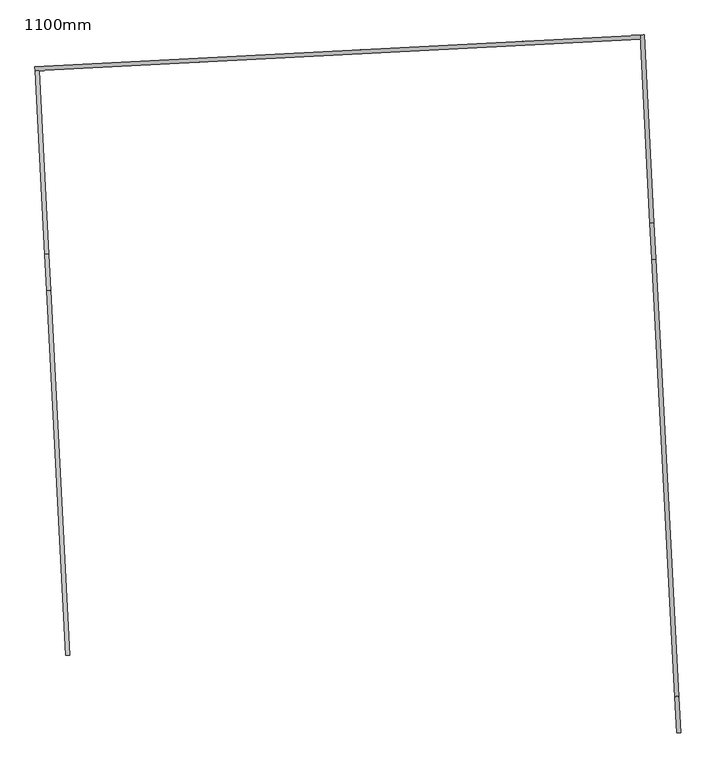
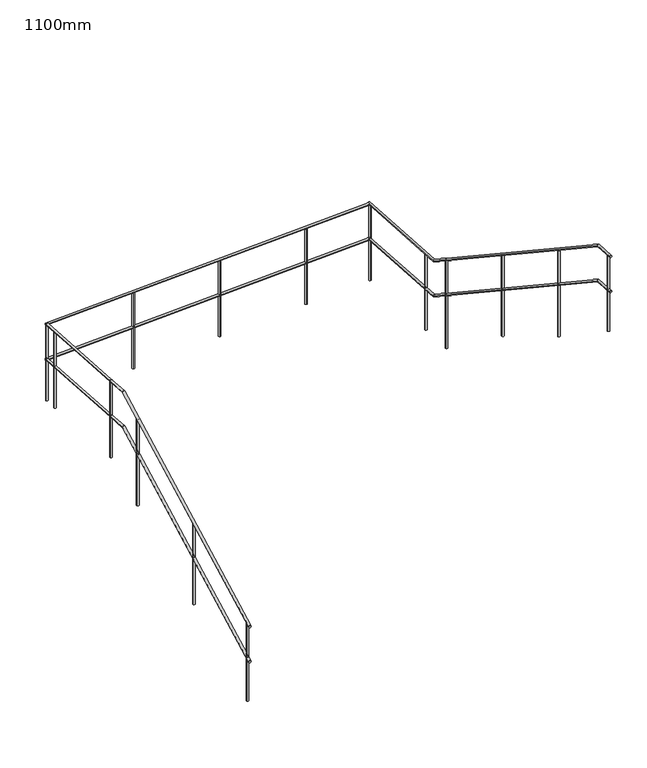
"""IFC4 building model written with IfcOpenShell, lengths in millimetres: railing geometry, 1100mm."""

from ifc_helpers import new_model, si_unit, point, frame, frame_2d, origin, place, context, project, spatial, circle_curve, ellipse_curve, trimmed, segment, composite_curve, outline, extrude, source, transform, mapped, element, save
from ifc_brep_helpers import plane_surface, cylinder_surface, advanced_brep


def railing_1100mm_925ff370(model_context):
    return source(origin(), model_context, "Body", "SolidModel", [
        advanced_brep(
        [(21553.8210897, 12464.3641407, 457.1248327), (21523.8622036, 12462.794062, 457.1248327), (21412.281847, 15165.0937775, 2210.0), (21382.3229609, 15163.5236988, 2210.0), (21398.3832997, 15430.2938589, 2210.0), (21368.4244136, 15428.7237802, 2210.0)],
        [
            (0, 1, ellipse_curve(frame((21538.8416467, 12463.5791013, 457.1248327), z_axis=(0.052335956242941364, -0.998629534754574, 0.0), x_axis=(0.0, 0.0, -1.0)), 17.8751673, 15.0)),
            (1, 0, ellipse_curve(frame((21538.8416467, 12463.5791013, 457.1248327), z_axis=(0.052335956242941364, -0.998629534754574, 0.0), x_axis=(0.0, 0.0, -1.0)), 17.8751673, 15.0)),
            (0, 2),
            (2, 3, ellipse_curve(frame((21397.302404, 15164.3087382, 2210.0), z_axis=(0.05018733030882, -0.957631309614881, -0.28359038545367027), x_axis=(-0.014841974004008681, 0.2832017346864693, -0.9589455111101147)), 15.6421818, 15.0)),
            (3, 1),
            (3, 2, ellipse_curve(frame((21397.302404, 15164.3087382, 2210.0), z_axis=(0.05018733030882, -0.957631309614881, -0.28359038545367027), x_axis=(-0.014841974004008681, 0.2832017346864693, -0.9589455111101147)), 15.6421818, 15.0)),
            (4, 5, circle_curve(frame((21383.4038566, 15429.5088195, 2210.0), z_axis=(-0.05233595624293373, 0.9986295347545745, 0.0), x_axis=(-0.9986295347545745, -0.05233595624293373, 0.0)), 15.0)),
            (5, 4, circle_curve(frame((21383.4038566, 15429.5088195, 2210.0), z_axis=(-0.05233595624293373, 0.9986295347545745, 0.0), x_axis=(-0.9986295347545745, -0.05233595624293373, 0.0)), 15.0)),
            (2, 4),
            (5, 3),
        ],
        [
            plane_surface(frame((21538.8416467, 12463.5791013, 475.0), z_axis=(0.052335956242941364, -0.998629534754574, 0.0), x_axis=(0.998629534754574, 0.052335956242941364, 0.0))),
            cylinder_surface(frame((21538.4146673, 12471.7263523, 462.4127052), z_axis=(0.04391787398555335, -0.8380029565528062, -0.5438954542495688), x_axis=(-0.998629534754574, -0.05233595624294136, 0.0)), 15.0),
            plane_surface(frame((21383.4038566, 15429.5088195, 2225.0), z_axis=(-0.05233595624293375, 0.9986295347545745, 0.0), x_axis=(0.9986295347545745, 0.05233595624293375, 0.0))),
            cylinder_surface(frame((21397.5345648, 15159.8788452, 2210.0), z_axis=(0.05233595624293373, -0.9986295347545745, 0.0), x_axis=(-0.9986295347545745, -0.05233595624293373, 0.0)), 15.0),
        ],
        [
            (0, [[1, 2]]),
            (1, [[-1, 3, 4, 5]]),
            (1, [[-2, -5, 6, -3]]),
            (2, [[7, 8]]),
            (3, [[-4, 9, -8, 10]]),
            (3, [[-6, -10, -7, -9]]),
        ],
    ),
        advanced_brep(
        [(21398.3832997, 15430.2938589, 2210.0), (21368.4244136, 15428.7237802, 2210.0), (21327.2273335, 16788.0305743, 2210.0), (21297.2684475, 16786.4604957, 2210.0)],
        [
            (0, 1, circle_curve(frame((21383.4038566, 15429.5088195, 2210.0), z_axis=(0.05233595624294149, -0.998629534754574, 0.0), x_axis=(-0.998629534754574, -0.05233595624294149, 0.0)), 15.0)),
            (1, 0, circle_curve(frame((21383.4038566, 15429.5088195, 2210.0), z_axis=(0.05233595624294149, -0.998629534754574, 0.0), x_axis=(-0.998629534754574, -0.05233595624294149, 0.0)), 15.0)),
            (2, 3, circle_curve(frame((21312.2478905, 16787.245535, 2210.0), z_axis=(-0.05233595624294149, 0.998629534754574, 0.0), x_axis=(-0.998629534754574, -0.05233595624294149, 0.0)), 15.0)),
            (3, 2, circle_curve(frame((21312.2478905, 16787.245535, 2210.0), z_axis=(-0.05233595624294149, 0.998629534754574, 0.0), x_axis=(-0.998629534754574, -0.05233595624294149, 0.0)), 15.0)),
            (0, 2),
            (3, 1),
        ],
        [
            plane_surface(frame((21383.4038566, 15429.5088195, 2225.0), z_axis=(0.05233595624294149, -0.998629534754574, 0.0), x_axis=(0.998629534754574, 0.05233595624294149, 0.0))),
            plane_surface(frame((21312.2478905, 16787.245535, 2225.0), z_axis=(-0.05233595624294221, 0.998629534754574, 0.0), x_axis=(0.998629534754574, 0.05233595624294221, 0.0))),
            cylinder_surface(frame((21383.4038566, 15429.5088195, 2210.0), z_axis=(0.05233595624294149, -0.998629534754574, 0.0), x_axis=(-0.998629534754574, -0.05233595624294149, 0.0)), 15.0),
        ],
        [
            (0, [[1, 2]]),
            (1, [[3, 4]]),
            (2, [[-1, 5, -4, 6]]),
            (2, [[-2, -6, -3, -5]]),
        ],
    ),
        advanced_brep(
        [(21297.2684475, 16786.4604957, 2210.0), (21295.6983688, 16816.4193817, 2210.0), (25777.8195811, 17021.2762305, 2210.0), (25776.2495024, 17051.2351166, 2210.0)],
        [
            (0, 1, circle_curve(frame((21296.4834082, 16801.4399387, 2210.0), z_axis=(-0.998629534754574, -0.05233595624294222, 0.0), x_axis=(-0.05233595624294222, 0.998629534754574, 0.0)), 15.0)),
            (1, 0, circle_curve(frame((21296.4834082, 16801.4399387, 2210.0), z_axis=(-0.998629534754574, -0.05233595624294222, 0.0), x_axis=(-0.05233595624294222, 0.998629534754574, 0.0)), 15.0)),
            (2, 3, circle_curve(frame((25777.0345417, 17036.2556736, 2210.0), z_axis=(0.998629534754574, 0.05233595624294222, 0.0), x_axis=(-0.05233595624294222, 0.998629534754574, 0.0)), 15.0)),
            (3, 2, circle_curve(frame((25777.0345417, 17036.2556736, 2210.0), z_axis=(0.998629534754574, 0.05233595624294222, 0.0), x_axis=(-0.05233595624294222, 0.998629534754574, 0.0)), 15.0)),
            (0, 2),
            (3, 1),
        ],
        [
            plane_surface(frame((21296.4834082, 16801.4399387, 2225.0), z_axis=(-0.998629534754574, -0.05233595624294149, 0.0), x_axis=(0.05233595624294149, -0.998629534754574, 0.0))),
            plane_surface(frame((25777.0345417, 17036.2556736, 2225.0), z_axis=(0.9986295347545739, 0.05233595624294333, 0.0), x_axis=(0.05233595624294333, -0.9986295347545739, 0.0))),
            cylinder_surface(frame((21296.4834082, 16801.4399387, 2210.0), z_axis=(-0.998629534754574, -0.05233595624294222, 0.0), x_axis=(-0.05233595624294222, 0.998629534754574, 0.0)), 15.0),
        ],
        [
            (0, [[1, 2]]),
            (1, [[3, 4]]),
            (2, [[-1, 5, -4, 6]]),
            (2, [[-2, -6, -3, -5]]),
        ],
    ),
        advanced_brep(
        [(25776.2495024, 17051.2351166, 2210.0), (25806.2083884, 17052.8051953, 2210.0), (25849.207708, 15659.1096221, 2210.0), (25879.1665941, 15660.6797008, 2210.0), (25863.1062554, 15393.9095407, 2382.1248327), (25893.0651414, 15395.4796194, 2382.1248327)],
        [
            (0, 1, circle_curve(frame((25791.2289454, 17052.0201559, 2210.0), z_axis=(-0.05233595624294333, 0.9986295347545739, 0.0), x_axis=(0.9986295347545739, 0.05233595624294333, 0.0)), 15.0)),
            (1, 0, circle_curve(frame((25791.2289454, 17052.0201559, 2210.0), z_axis=(-0.05233595624294333, 0.9986295347545739, 0.0), x_axis=(0.9986295347545739, 0.05233595624294333, 0.0)), 15.0)),
            (0, 2),
            (2, 3, ellipse_curve(frame((25864.1871511, 15659.8946614, 2210.0), z_axis=(-0.05018733030882886, 0.9576313096148807, -0.2835903854536695), x_axis=(-0.014841974004012624, 0.28320173468646914, 0.9589455111101145)), 15.6421818, 15.0)),
            (3, 1),
            (3, 2, ellipse_curve(frame((25864.1871511, 15659.8946614, 2210.0), z_axis=(-0.05018733030882886, 0.9576313096148807, -0.2835903854536695), x_axis=(-0.014841974004012624, 0.28320173468646914, 0.9589455111101145)), 15.6421818, 15.0)),
            (4, 5, ellipse_curve(frame((25878.0856984, 15394.69458, 2382.1248327), z_axis=(0.05233595624295016, -0.9986295347545736, 0.0), x_axis=(0.0, 0.0, -1.0)), 17.8751673, 15.0)),
            (5, 4, ellipse_curve(frame((25878.0856984, 15394.69458, 2382.1248327), z_axis=(0.05233595624295016, -0.9986295347545736, 0.0), x_axis=(0.0, 0.0, -1.0)), 17.8751673, 15.0)),
            (2, 4),
            (5, 3),
        ],
        [
            plane_surface(frame((25791.2289454, 17052.0201559, 2225.0), z_axis=(-0.05233595624294221, 0.998629534754574, 0.0), x_axis=(0.998629534754574, 0.05233595624294221, 0.0))),
            cylinder_surface(frame((25791.2289454, 17052.0201559, 2210.0), z_axis=(-0.05233595624294333, 0.9986295347545739, 0.0), x_axis=(0.9986295347545739, 0.05233595624294333, 0.0)), 15.0),
            plane_surface(frame((25878.0856984, 15394.69458, 2400.0), z_axis=(0.05233595624295016, -0.9986295347545736, 0.0), x_axis=(0.9986295347545736, 0.05233595624295016, 0.0))),
            cylinder_surface(frame((25864.3819695, 15656.1773035, 2212.4127052), z_axis=(-0.043917873985560775, 0.838002956552807, -0.5438954542495672), x_axis=(0.9986295347545737, 0.05233595624294905, 0.0)), 15.0),
        ],
        [
            (0, [[1, 2]]),
            (1, [[-1, 3, 4, 5]]),
            (1, [[-2, -5, 6, -3]]),
            (2, [[7, 8]]),
            (3, [[-4, 9, -8, 10]]),
            (3, [[-6, -10, -7, -9]]),
        ],
    ),
        advanced_brep(
        [(25863.1062554, 15393.9095407, 2382.1248327), (25893.0651414, 15395.4796194, 2382.1248327), (26032.9069145, 12153.9199551, 4485.0), (26062.8658005, 12155.4900338, 4485.0), (26046.8054618, 11888.7198737, 4485.0), (26076.7643478, 11890.2899524, 4485.0)],
        [
            (0, 1, ellipse_curve(frame((25878.0856984, 15394.69458, 2382.1248327), z_axis=(-0.052335956242941906, 0.998629534754574, 0.0), x_axis=(0.0, 0.0, -1.0)), 17.8751673, 15.0)),
            (1, 0, ellipse_curve(frame((25878.0856984, 15394.69458, 2382.1248327), z_axis=(-0.052335956242941906, 0.998629534754574, 0.0), x_axis=(0.0, 0.0, -1.0)), 17.8751673, 15.0)),
            (0, 2),
            (2, 3, ellipse_curve(frame((26047.8863575, 12154.7049944, 4485.0), z_axis=(-0.05018733030882246, 0.957631309614881, -0.28359038545366994), x_axis=(0.01484197400401534, -0.2832017346864691, -0.9589455111101146)), 15.6421818, 15.0)),
            (3, 1),
            (3, 2, ellipse_curve(frame((26047.8863575, 12154.7049944, 4485.0), z_axis=(-0.05018733030882246, 0.957631309614881, -0.28359038545366994), x_axis=(0.01484197400401534, -0.2832017346864691, -0.9589455111101146)), 15.6421818, 15.0)),
            (4, 5, circle_curve(frame((26061.7849048, 11889.5049131, 4485.0), z_axis=(0.05233595624293795, -0.9986295347545743, 0.0), x_axis=(0.9986295347545743, 0.05233595624293795, 0.0)), 15.0)),
            (5, 4, circle_curve(frame((26061.7849048, 11889.5049131, 4485.0), z_axis=(0.05233595624293795, -0.9986295347545743, 0.0), x_axis=(0.9986295347545743, 0.05233595624293795, 0.0)), 15.0)),
            (2, 4),
            (5, 3),
        ],
        [
            plane_surface(frame((25878.0856984, 15394.69458, 2400.0), z_axis=(-0.052335956242941906, 0.998629534754574, 0.0), x_axis=(0.998629534754574, 0.052335956242941906, 0.0))),
            cylinder_surface(frame((25878.5126777, 15386.5473291, 2387.4127052), z_axis=(-0.04391787398555386, 0.8380029565528069, -0.5438954542495675), x_axis=(0.998629534754574, 0.05233595624294191, 0.0)), 15.0),
            plane_surface(frame((26061.7849048, 11889.5049131, 4500.0), z_axis=(0.05233595624293795, -0.9986295347545743, 0.0), x_axis=(0.9986295347545743, 0.05233595624293795, 0.0))),
            cylinder_surface(frame((26047.6541966, 12159.1348874, 4485.0), z_axis=(-0.05233595624293795, 0.9986295347545743, 0.0), x_axis=(0.9986295347545743, 0.05233595624293795, 0.0)), 15.0),
        ],
        [
            (0, [[1, 2]]),
            (1, [[-1, 3, 4, 5]]),
            (1, [[-2, -5, 6, -3]]),
            (2, [[7, 8]]),
            (3, [[-4, 9, -8, 10]]),
            (3, [[-6, -10, -7, -9]]),
        ],
    ),
        advanced_brep(
        [(21553.8210897, 12464.3641407, 957.1248327), (21523.8622036, 12462.794062, 957.1248327), (21412.281847, 15165.0937775, 2710.0), (21382.3229609, 15163.5236988, 2710.0), (21398.3832997, 15430.2938589, 2710.0), (21368.4244136, 15428.7237802, 2710.0)],
        [
            (0, 1, ellipse_curve(frame((21538.8416467, 12463.5791013, 957.1248327), z_axis=(0.052335956242941364, -0.998629534754574, 0.0), x_axis=(0.0, 0.0, -1.0)), 17.8751673, 15.0)),
            (1, 0, ellipse_curve(frame((21538.8416467, 12463.5791013, 957.1248327), z_axis=(0.052335956242941364, -0.998629534754574, 0.0), x_axis=(0.0, 0.0, -1.0)), 17.8751673, 15.0)),
            (0, 2),
            (2, 3, ellipse_curve(frame((21397.302404, 15164.3087382, 2710.0), z_axis=(0.05018733030882, -0.957631309614881, -0.28359038545367027), x_axis=(-0.014841974004008681, 0.2832017346864693, -0.9589455111101147)), 15.6421818, 15.0)),
            (3, 1),
            (3, 2, ellipse_curve(frame((21397.302404, 15164.3087382, 2710.0), z_axis=(0.05018733030882, -0.957631309614881, -0.28359038545367027), x_axis=(-0.014841974004008681, 0.2832017346864693, -0.9589455111101147)), 15.6421818, 15.0)),
            (4, 5, circle_curve(frame((21383.4038566, 15429.5088195, 2710.0), z_axis=(-0.05233595624293373, 0.9986295347545745, 0.0), x_axis=(-0.9986295347545745, -0.05233595624293373, 0.0)), 15.0)),
            (5, 4, circle_curve(frame((21383.4038566, 15429.5088195, 2710.0), z_axis=(-0.05233595624293373, 0.9986295347545745, 0.0), x_axis=(-0.9986295347545745, -0.05233595624293373, 0.0)), 15.0)),
            (2, 4),
            (5, 3),
        ],
        [
            plane_surface(frame((21538.8416467, 12463.5791013, 975.0), z_axis=(0.052335956242941364, -0.998629534754574, 0.0), x_axis=(0.998629534754574, 0.052335956242941364, 0.0))),
            cylinder_surface(frame((21538.4146673, 12471.7263523, 962.4127052), z_axis=(0.04391787398555335, -0.8380029565528062, -0.5438954542495688), x_axis=(-0.998629534754574, -0.05233595624294136, 0.0)), 15.0),
            plane_surface(frame((21383.4038566, 15429.5088195, 2725.0), z_axis=(-0.05233595624293375, 0.9986295347545745, 0.0), x_axis=(0.9986295347545745, 0.05233595624293375, 0.0))),
            cylinder_surface(frame((21397.5345648, 15159.8788452, 2710.0), z_axis=(0.05233595624293373, -0.9986295347545745, 0.0), x_axis=(-0.9986295347545745, -0.05233595624293373, 0.0)), 15.0),
        ],
        [
            (0, [[1, 2]]),
            (1, [[-1, 3, 4, 5]]),
            (1, [[-2, -5, 6, -3]]),
            (2, [[7, 8]]),
            (3, [[-4, 9, -8, 10]]),
            (3, [[-6, -10, -7, -9]]),
        ],
    ),
        advanced_brep(
        [(21398.3832997, 15430.2938589, 2710.0), (21368.4244136, 15428.7237802, 2710.0), (21327.2273335, 16788.0305743, 2710.0), (21297.2684475, 16786.4604957, 2710.0)],
        [
            (0, 1, circle_curve(frame((21383.4038566, 15429.5088195, 2710.0), z_axis=(0.05233595624294149, -0.998629534754574, 0.0), x_axis=(-0.998629534754574, -0.05233595624294149, 0.0)), 15.0)),
            (1, 0, circle_curve(frame((21383.4038566, 15429.5088195, 2710.0), z_axis=(0.05233595624294149, -0.998629534754574, 0.0), x_axis=(-0.998629534754574, -0.05233595624294149, 0.0)), 15.0)),
            (2, 3, circle_curve(frame((21312.2478905, 16787.245535, 2710.0), z_axis=(-0.05233595624294149, 0.998629534754574, 0.0), x_axis=(-0.998629534754574, -0.05233595624294149, 0.0)), 15.0)),
            (3, 2, circle_curve(frame((21312.2478905, 16787.245535, 2710.0), z_axis=(-0.05233595624294149, 0.998629534754574, 0.0), x_axis=(-0.998629534754574, -0.05233595624294149, 0.0)), 15.0)),
            (0, 2),
            (3, 1),
        ],
        [
            plane_surface(frame((21383.4038566, 15429.5088195, 2725.0), z_axis=(0.05233595624294149, -0.998629534754574, 0.0), x_axis=(0.998629534754574, 0.05233595624294149, 0.0))),
            plane_surface(frame((21312.2478905, 16787.245535, 2725.0), z_axis=(-0.05233595624294221, 0.998629534754574, 0.0), x_axis=(0.998629534754574, 0.05233595624294221, 0.0))),
            cylinder_surface(frame((21383.4038566, 15429.5088195, 2710.0), z_axis=(0.05233595624294149, -0.998629534754574, 0.0), x_axis=(-0.998629534754574, -0.05233595624294149, 0.0)), 15.0),
        ],
        [
            (0, [[1, 2]]),
            (1, [[3, 4]]),
            (2, [[-1, 5, -4, 6]]),
            (2, [[-2, -6, -3, -5]]),
        ],
    ),
        advanced_brep(
        [(21297.2684475, 16786.4604957, 2710.0), (21295.6983688, 16816.4193817, 2710.0), (25777.8195811, 17021.2762305, 2710.0), (25776.2495024, 17051.2351166, 2710.0)],
        [
            (0, 1, circle_curve(frame((21296.4834082, 16801.4399387, 2710.0), z_axis=(-0.998629534754574, -0.05233595624294222, 0.0), x_axis=(-0.05233595624294222, 0.998629534754574, 0.0)), 15.0)),
            (1, 0, circle_curve(frame((21296.4834082, 16801.4399387, 2710.0), z_axis=(-0.998629534754574, -0.05233595624294222, 0.0), x_axis=(-0.05233595624294222, 0.998629534754574, 0.0)), 15.0)),
            (2, 3, circle_curve(frame((25777.0345417, 17036.2556736, 2710.0), z_axis=(0.998629534754574, 0.05233595624294222, 0.0), x_axis=(-0.05233595624294222, 0.998629534754574, 0.0)), 15.0)),
            (3, 2, circle_curve(frame((25777.0345417, 17036.2556736, 2710.0), z_axis=(0.998629534754574, 0.05233595624294222, 0.0), x_axis=(-0.05233595624294222, 0.998629534754574, 0.0)), 15.0)),
            (0, 2),
            (3, 1),
        ],
        [
            plane_surface(frame((21296.4834082, 16801.4399387, 2725.0), z_axis=(-0.998629534754574, -0.05233595624294149, 0.0), x_axis=(0.05233595624294149, -0.998629534754574, 0.0))),
            plane_surface(frame((25777.0345417, 17036.2556736, 2725.0), z_axis=(0.9986295347545739, 0.05233595624294333, 0.0), x_axis=(0.05233595624294333, -0.9986295347545739, 0.0))),
            cylinder_surface(frame((21296.4834082, 16801.4399387, 2710.0), z_axis=(-0.998629534754574, -0.05233595624294222, 0.0), x_axis=(-0.05233595624294222, 0.998629534754574, 0.0)), 15.0),
        ],
        [
            (0, [[1, 2]]),
            (1, [[3, 4]]),
            (2, [[-1, 5, -4, 6]]),
            (2, [[-2, -6, -3, -5]]),
        ],
    ),
        advanced_brep(
        [(25776.2495024, 17051.2351166, 2710.0), (25806.2083884, 17052.8051953, 2710.0), (25849.207708, 15659.1096221, 2710.0), (25879.1665941, 15660.6797008, 2710.0), (25863.1062554, 15393.9095407, 2882.1248327), (25893.0651414, 15395.4796194, 2882.1248327)],
        [
            (0, 1, circle_curve(frame((25791.2289454, 17052.0201559, 2710.0), z_axis=(-0.05233595624294333, 0.9986295347545739, 0.0), x_axis=(0.9986295347545739, 0.05233595624294333, 0.0)), 15.0)),
            (1, 0, circle_curve(frame((25791.2289454, 17052.0201559, 2710.0), z_axis=(-0.05233595624294333, 0.9986295347545739, 0.0), x_axis=(0.9986295347545739, 0.05233595624294333, 0.0)), 15.0)),
            (0, 2),
            (2, 3, ellipse_curve(frame((25864.1871511, 15659.8946614, 2710.0), z_axis=(-0.05018733030882886, 0.9576313096148807, -0.2835903854536695), x_axis=(-0.014841974004012624, 0.28320173468646914, 0.9589455111101145)), 15.6421818, 15.0)),
            (3, 1),
            (3, 2, ellipse_curve(frame((25864.1871511, 15659.8946614, 2710.0), z_axis=(-0.05018733030882886, 0.9576313096148807, -0.2835903854536695), x_axis=(-0.014841974004012624, 0.28320173468646914, 0.9589455111101145)), 15.6421818, 15.0)),
            (4, 5, ellipse_curve(frame((25878.0856984, 15394.69458, 2882.1248327), z_axis=(0.05233595624295016, -0.9986295347545736, 0.0), x_axis=(0.0, 0.0, -1.0)), 17.8751673, 15.0)),
            (5, 4, ellipse_curve(frame((25878.0856984, 15394.69458, 2882.1248327), z_axis=(0.05233595624295016, -0.9986295347545736, 0.0), x_axis=(0.0, 0.0, -1.0)), 17.8751673, 15.0)),
            (2, 4),
            (5, 3),
        ],
        [
            plane_surface(frame((25791.2289454, 17052.0201559, 2725.0), z_axis=(-0.05233595624294221, 0.998629534754574, 0.0), x_axis=(0.998629534754574, 0.05233595624294221, 0.0))),
            cylinder_surface(frame((25791.2289454, 17052.0201559, 2710.0), z_axis=(-0.05233595624294333, 0.9986295347545739, 0.0), x_axis=(0.9986295347545739, 0.05233595624294333, 0.0)), 15.0),
            plane_surface(frame((25878.0856984, 15394.69458, 2900.0), z_axis=(0.05233595624295016, -0.9986295347545736, 0.0), x_axis=(0.9986295347545736, 0.05233595624295016, 0.0))),
            cylinder_surface(frame((25864.3819695, 15656.1773035, 2712.4127052), z_axis=(-0.043917873985560775, 0.838002956552807, -0.5438954542495672), x_axis=(0.9986295347545737, 0.05233595624294905, 0.0)), 15.0),
        ],
        [
            (0, [[1, 2]]),
            (1, [[-1, 3, 4, 5]]),
            (1, [[-2, -5, 6, -3]]),
            (2, [[7, 8]]),
            (3, [[-4, 9, -8, 10]]),
            (3, [[-6, -10, -7, -9]]),
        ],
    ),
        advanced_brep(
        [(25863.1062554, 15393.9095407, 2882.1248327), (25893.0651414, 15395.4796194, 2882.1248327), (26032.9069145, 12153.9199551, 4985.0), (26062.8658005, 12155.4900338, 4985.0), (26046.8054618, 11888.7198737, 4985.0), (26076.7643478, 11890.2899524, 4985.0)],
        [
            (0, 1, ellipse_curve(frame((25878.0856984, 15394.69458, 2882.1248327), z_axis=(-0.052335956242941906, 0.998629534754574, 0.0), x_axis=(0.0, 0.0, -1.0)), 17.8751673, 15.0)),
            (1, 0, ellipse_curve(frame((25878.0856984, 15394.69458, 2882.1248327), z_axis=(-0.052335956242941906, 0.998629534754574, 0.0), x_axis=(0.0, 0.0, -1.0)), 17.8751673, 15.0)),
            (0, 2),
            (2, 3, ellipse_curve(frame((26047.8863575, 12154.7049944, 4985.0), z_axis=(-0.05018733030882246, 0.957631309614881, -0.28359038545366994), x_axis=(0.01484197400401534, -0.2832017346864691, -0.9589455111101146)), 15.6421818, 15.0)),
            (3, 1),
            (3, 2, ellipse_curve(frame((26047.8863575, 12154.7049944, 4985.0), z_axis=(-0.05018733030882246, 0.957631309614881, -0.28359038545366994), x_axis=(0.01484197400401534, -0.2832017346864691, -0.9589455111101146)), 15.6421818, 15.0)),
            (4, 5, circle_curve(frame((26061.7849048, 11889.5049131, 4985.0), z_axis=(0.05233595624293795, -0.9986295347545743, 0.0), x_axis=(0.9986295347545743, 0.05233595624293795, 0.0)), 15.0)),
            (5, 4, circle_curve(frame((26061.7849048, 11889.5049131, 4985.0), z_axis=(0.05233595624293795, -0.9986295347545743, 0.0), x_axis=(0.9986295347545743, 0.05233595624293795, 0.0)), 15.0)),
            (2, 4),
            (5, 3),
        ],
        [
            plane_surface(frame((25878.0856984, 15394.69458, 2900.0), z_axis=(-0.052335956242941906, 0.998629534754574, 0.0), x_axis=(0.998629534754574, 0.052335956242941906, 0.0))),
            cylinder_surface(frame((25878.5126777, 15386.5473291, 2887.4127052), z_axis=(-0.04391787398555386, 0.8380029565528069, -0.5438954542495675), x_axis=(0.998629534754574, 0.05233595624294191, 0.0)), 15.0),
            plane_surface(frame((26061.7849048, 11889.5049131, 5000.0), z_axis=(0.05233595624293795, -0.9986295347545743, 0.0), x_axis=(0.9986295347545743, 0.05233595624293795, 0.0))),
            cylinder_surface(frame((26047.6541966, 12159.1348874, 4985.0), z_axis=(-0.05233595624293795, 0.9986295347545743, 0.0), x_axis=(0.9986295347545743, 0.05233595624293795, 0.0)), 15.0),
        ],
        [
            (0, [[1, 2]]),
            (1, [[-1, 3, 4, 5]]),
            (1, [[-2, -5, 6, -3]]),
            (2, [[7, 8]]),
            (3, [[-4, 9, -8, 10]]),
            (3, [[-6, -10, -7, -9]]),
        ],
    ),
        extrude(outline(composite_curve([segment(trimmed(circle_curve(frame_2d((26003.6919934, 12997.9836966)), 15.0), [point((26018.6714364, 12998.768736))], [point((25988.7125504, 12997.1986573))], False, "CARTESIAN"), True, "CONTINUOUS"), segment(trimmed(circle_curve(frame_2d((26003.6919934, 12997.9836966)), 15.0), [point((25988.7125504, 12997.1986573))], [point((26018.6714364, 12998.768736))], False, "CARTESIAN"), True, "CONTINUOUS")], self_intersect=False)), frame((0.0, 0.0, 3200.0), z_axis=(0.0, 0.0, 1.0), x_axis=(1.0, 0.0, 0.0)), (0.0, 0.0, 1.0), 1225.5555556),
        extrude(outline(composite_curve([segment(trimmed(circle_curve(frame_2d((25940.8888459, 14196.3391383)), 15.0), [point((25955.8682889, 14197.1241777))], [point((25925.9094029, 14195.554099))], False, "CARTESIAN"), True, "CONTINUOUS"), segment(trimmed(circle_curve(frame_2d((25940.8888459, 14196.3391383)), 15.0), [point((25925.9094029, 14195.554099))], [point((25955.8682889, 14197.1241777))], False, "CARTESIAN"), True, "CONTINUOUS")], self_intersect=False)), frame((0.0, 0.0, 2500.0), z_axis=(0.0, 0.0, 1.0), x_axis=(1.0, 0.0, 0.0)), (0.0, 0.0, 1.0), 1147.7777778),
        extrude(outline(composite_curve([segment(trimmed(circle_curve(frame_2d((25854.8171323, 15838.6852712)), 15.0), [point((25869.7965753, 15839.4703105))], [point((25839.8376892, 15837.9002318))], False, "CARTESIAN"), True, "CONTINUOUS"), segment(trimmed(circle_curve(frame_2d((25854.8171323, 15838.6852712)), 15.0), [point((25839.8376892, 15837.9002318))], [point((25869.7965753, 15839.4703105))], False, "CARTESIAN"), True, "CONTINUOUS")], self_intersect=False)), frame((0.0, 0.0, 1625.0), z_axis=(0.0, 0.0, 1.0), x_axis=(1.0, 0.0, 0.0)), (0.0, 0.0, 1.0), 1070.0),
        extrude(outline(composite_curve([segment(trimmed(circle_curve(frame_2d((24906.5291763, 16990.6344205)), 15.0), [point((24905.744137, 17005.6138635))], [point((24907.3142156, 16975.6549775))], False, "CARTESIAN"), True, "CONTINUOUS"), segment(trimmed(circle_curve(frame_2d((24906.5291763, 16990.6344205)), 15.0), [point((24907.3142156, 16975.6549775))], [point((24905.744137, 17005.6138635))], False, "CARTESIAN"), True, "CONTINUOUS")], self_intersect=False)), frame((0.0, 0.0, 1625.0), z_axis=(0.0, 0.0, 1.0), x_axis=(1.0, 0.0, 0.0)), (0.0, 0.0, 1.0), 1070.0),
        extrude(outline(composite_curve([segment(trimmed(circle_curve(frame_2d((23708.1737346, 16927.831273)), 15.0), [point((23707.3886952, 16942.810716))], [point((23708.9587739, 16912.85183))], False, "CARTESIAN"), True, "CONTINUOUS"), segment(trimmed(circle_curve(frame_2d((23708.1737346, 16927.831273)), 15.0), [point((23708.9587739, 16912.85183))], [point((23707.3886952, 16942.810716))], False, "CARTESIAN"), True, "CONTINUOUS")], self_intersect=False)), frame((0.0, 0.0, 1625.0), z_axis=(0.0, 0.0, 1.0), x_axis=(1.0, 0.0, 0.0)), (0.0, 0.0, 1.0), 1070.0),
        extrude(outline(composite_curve([segment(trimmed(circle_curve(frame_2d((22509.8182929, 16865.0281255)), 15.0), [point((22509.0332535, 16880.0075685))], [point((22510.6033322, 16850.0486825))], False, "CARTESIAN"), True, "CONTINUOUS"), segment(trimmed(circle_curve(frame_2d((22509.8182929, 16865.0281255)), 15.0), [point((22510.6033322, 16850.0486825))], [point((22509.0332535, 16880.0075685))], False, "CARTESIAN"), True, "CONTINUOUS")], self_intersect=False)), frame((0.0, 0.0, 1625.0), z_axis=(0.0, 0.0, 1.0), x_axis=(1.0, 0.0, 0.0)), (0.0, 0.0, 1.0), 1070.0),
        extrude(outline(composite_curve([segment(trimmed(circle_curve(frame_2d((21320.6007091, 16627.8642613)), 15.0), [point((21305.6212661, 16627.0792219))], [point((21335.5801522, 16628.6493006))], False, "CARTESIAN"), True, "CONTINUOUS"), segment(trimmed(circle_curve(frame_2d((21320.6007091, 16627.8642613)), 15.0), [point((21335.5801522, 16628.6493006))], [point((21305.6212661, 16627.0792219))], False, "CARTESIAN"), True, "CONTINUOUS")], self_intersect=False)), frame((0.0, 0.0, 1625.0), z_axis=(0.0, 0.0, 1.0), x_axis=(1.0, 0.0, 0.0)), (0.0, 0.0, 1.0), 1070.0),
        extrude(outline(composite_curve([segment(trimmed(circle_curve(frame_2d((21413.2353517, 14860.2899847)), 15.0), [point((21398.2559087, 14859.5049454))], [point((21428.2147947, 14861.0750241))], False, "CARTESIAN"), True, "CONTINUOUS"), segment(trimmed(circle_curve(frame_2d((21413.2353517, 14860.2899847)), 15.0), [point((21428.2147947, 14861.0750241))], [point((21398.2559087, 14859.5049454))], False, "CARTESIAN"), True, "CONTINUOUS")], self_intersect=False)), frame((0.0, 0.0, 1275.0), z_axis=(0.0, 0.0, 1.0), x_axis=(1.0, 0.0, 0.0)), (0.0, 0.0, 1.0), 1225.5555556),
        extrude(outline(composite_curve([segment(trimmed(circle_curve(frame_2d((21476.0384992, 13661.934543)), 15.0), [point((21461.0590562, 13661.1495037))], [point((21491.0179422, 13662.7195824))], False, "CARTESIAN"), True, "CONTINUOUS"), segment(trimmed(circle_curve(frame_2d((21476.0384992, 13661.934543)), 15.0), [point((21491.0179422, 13662.7195824))], [point((21461.0590562, 13661.1495037))], False, "CARTESIAN"), True, "CONTINUOUS")], self_intersect=False)), frame((0.0, 0.0, 575.0), z_axis=(0.0, 0.0, 1.0), x_axis=(1.0, 0.0, 0.0)), (0.0, 0.0, 1.0), 1147.7777778),
        extrude(outline(composite_curve([segment(trimmed(circle_curve(frame_2d((25878.0856984, 15394.69458)), 15.0), [point((25893.0651414, 15395.4796194))], [point((25863.1062554, 15393.9095407))], False, "CARTESIAN"), True, "CONTINUOUS"), segment(trimmed(circle_curve(frame_2d((25878.0856984, 15394.69458)), 15.0), [point((25863.1062554, 15393.9095407))], [point((25893.0651414, 15395.4796194))], False, "CARTESIAN"), True, "CONTINUOUS")], self_intersect=False)), frame((0.0, 0.0, 1625.0), z_axis=(0.0, 0.0, 1.0), x_axis=(1.0, 0.0, 0.0)), (0.0, 0.0, 1.0), 1245.0),
        extrude(outline(composite_curve([segment(trimmed(circle_curve(frame_2d((25792.0139848, 17037.0407129)), 15.0), [point((25791.2289454, 17052.0201559))], [point((25792.7990241, 17022.0612699))], False, "CARTESIAN"), True, "CONTINUOUS"), segment(trimmed(circle_curve(frame_2d((25792.0139848, 17037.0407129)), 15.0), [point((25792.7990241, 17022.0612699))], [point((25791.2289454, 17052.0201559))], False, "CARTESIAN"), True, "CONTINUOUS")], self_intersect=False)), frame((0.0, 0.0, 1625.0), z_axis=(0.0, 0.0, 1.0), x_axis=(1.0, 0.0, 0.0)), (0.0, 0.0, 1.0), 1070.0),
        extrude(outline(composite_curve([segment(trimmed(circle_curve(frame_2d((21311.4628512, 16802.224978)), 15.0), [point((21296.4834082, 16801.4399387))], [point((21326.4422942, 16803.0100174))], False, "CARTESIAN"), True, "CONTINUOUS"), segment(trimmed(circle_curve(frame_2d((21311.4628512, 16802.224978)), 15.0), [point((21326.4422942, 16803.0100174))], [point((21296.4834082, 16801.4399387))], False, "CARTESIAN"), True, "CONTINUOUS")], self_intersect=False)), frame((0.0, 0.0, 1625.0), z_axis=(0.0, 0.0, 1.0), x_axis=(1.0, 0.0, 0.0)), (0.0, 0.0, 1.0), 1070.0),
        extrude(outline(composite_curve([segment(trimmed(circle_curve(frame_2d((21383.4038566, 15429.5088195)), 15.0), [point((21368.4244136, 15428.7237802))], [point((21398.3832997, 15430.2938589))], False, "CARTESIAN"), True, "CONTINUOUS"), segment(trimmed(circle_curve(frame_2d((21383.4038566, 15429.5088195)), 15.0), [point((21398.3832997, 15430.2938589))], [point((21368.4244136, 15428.7237802))], False, "CARTESIAN"), True, "CONTINUOUS")], self_intersect=False)), frame((0.0, 0.0, 1625.0), z_axis=(0.0, 0.0, 1.0), x_axis=(1.0, 0.0, 0.0)), (0.0, 0.0, 1.0), 1070.0),
        extrude(outline(composite_curve([segment(trimmed(circle_curve(frame_2d((26059.168107, 11939.4363898)), 15.0), [point((26074.14755, 11940.2214291))], [point((26044.188664, 11938.6513504))], False, "CARTESIAN"), True, "CONTINUOUS"), segment(trimmed(circle_curve(frame_2d((26059.168107, 11939.4363898)), 15.0), [point((26044.188664, 11938.6513504))], [point((26074.14755, 11940.2214291))], False, "CARTESIAN"), True, "CONTINUOUS")], self_intersect=False)), frame((0.0, 0.0, 3900.0), z_axis=(0.0, 0.0, 1.0), x_axis=(1.0, 0.0, 0.0)), (0.0, 0.0, 1.0), 1070.0),
        extrude(outline(composite_curve([segment(trimmed(circle_curve(frame_2d((21536.2248489, 12513.5105781)), 15.0), [point((21521.2454058, 12512.7255387))], [point((21551.2042919, 12514.2956174))], False, "CARTESIAN"), True, "CONTINUOUS"), segment(trimmed(circle_curve(frame_2d((21536.2248489, 12513.5105781)), 15.0), [point((21551.2042919, 12514.2956174))], [point((21521.2454058, 12512.7255387))], False, "CARTESIAN"), True, "CONTINUOUS")], self_intersect=False)), frame((0.0, 0.0, -125.0), z_axis=(0.0, 0.0, 1.0), x_axis=(1.0, 0.0, 0.0)), (0.0, 0.0, 1.0), 1102.4074074),
    ])


if __name__ == "__main__":
    model = new_model("IFC4")
    model_context = context("Model", 3, world=origin())
    ifc_project = project(units=[si_unit("LENGTHUNIT", "METRE", prefix="MILLI")], contexts=[model_context])
    site = spatial("IfcSite", under=ifc_project)
    building = spatial("IfcBuilding", under=site)
    placement = place(None, origin())
    railing_1100mm_shape = railing_1100mm_925ff370(model_context)
    element("IfcRailing", 1, ObjectType="1100mm", at=placement, inside=building, context=model_context, shape_type="MappedRepresentation", body=[
        mapped(railing_1100mm_shape, transform((0.0, 0.0, 0.0), x_axis=(1.0, 0.0, 0.0), y_axis=(0.0, 1.0, 0.0), z_axis=(0.0, 0.0, 1.0))),
    ])
    save(model, "model.ifc")
